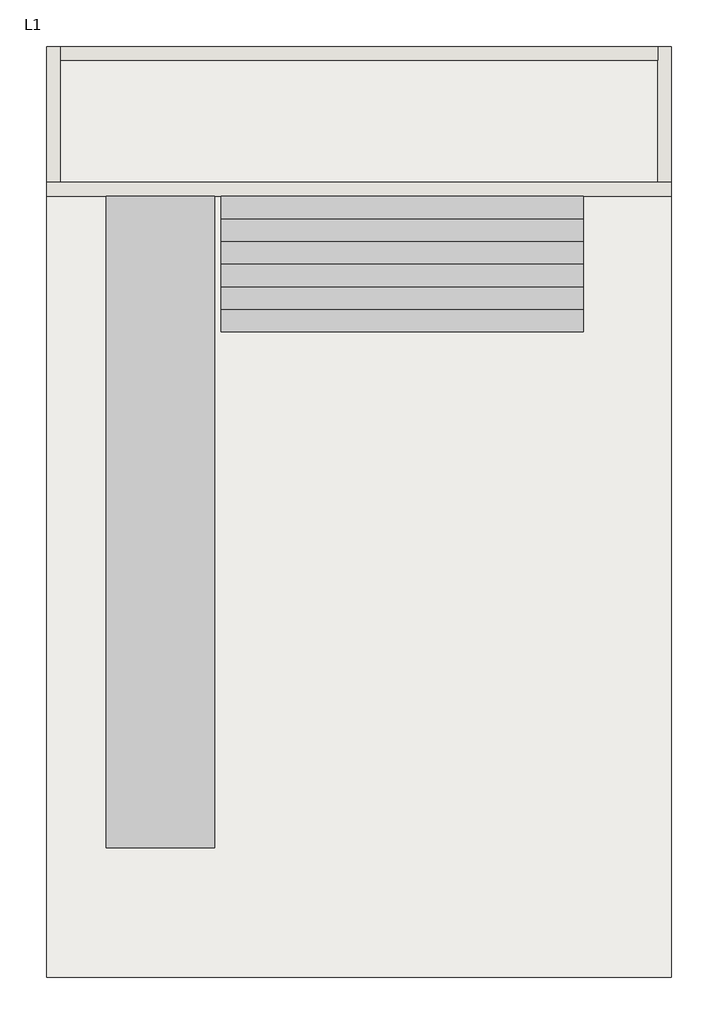
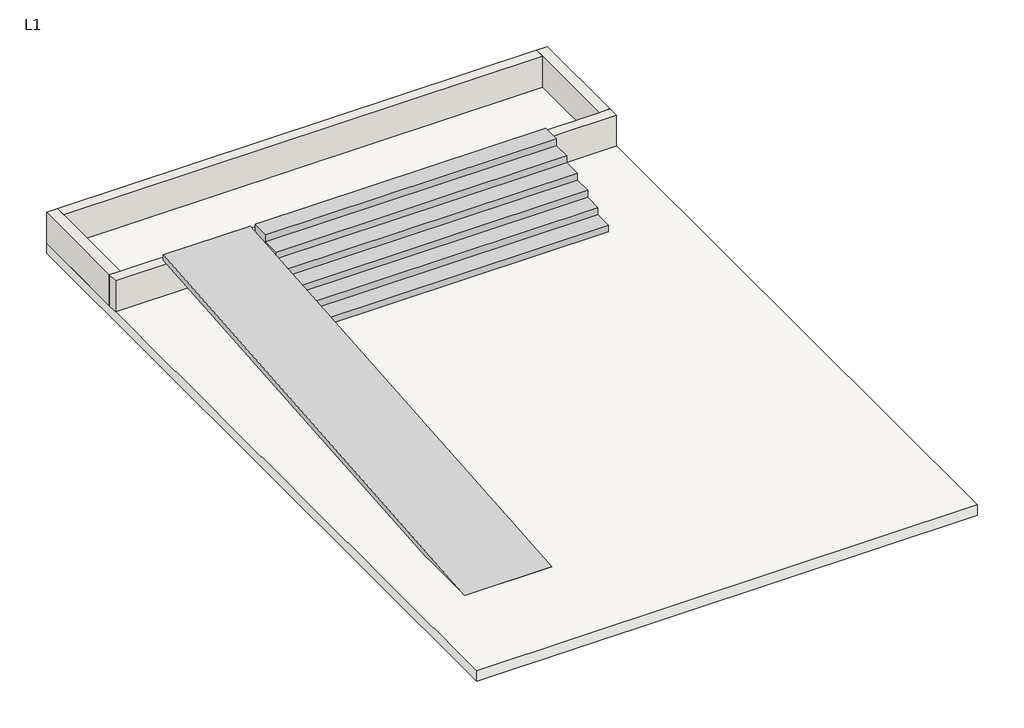
# One storey: 4 walls, 1 ramp, 1 slab, 1 stair flight.
"""IFC4 building model written with IfcOpenShell, lengths in millimetres."""

import ifcopenshell
import ifcopenshell.guid

model = None  # the IFC model being written
_history = None  # IfcOwnerHistory: only IFC2X3 demands one
_inside = {}  # id of a spatial element -> (the spatial element, [elements in it])
_under = {}  # id of a project, library or spatial element -> (it, [spatial elements below it])
_declared = {}  # id of a project -> (the project, [libraries it declares])
_typed = {}  # id of a type object -> (the type object, [elements of that type])
_made_of = {}  # id of a material, layer set ... -> (it, [elements and type objects made of it])


def new_model(schema):
    """Start an empty IFC model of exactly this schema.

    Asked for "IFC4X3", IfcOpenShell would pick the latest addendum, in which some entities
    have other attributes; the version numbers below select the first issue.
    IFC2X3 requires an IfcOwnerHistory on every rooted entity: one is made here for all.
    """
    global model, _history
    if schema == "IFC4X3":
        model = ifcopenshell.file(schema_version=(4, 3, 0, 0))
    else:
        model = ifcopenshell.file(schema=schema)
    _inside.clear()
    _under.clear()
    _declared.clear()
    _typed.clear()
    _made_of.clear()
    _history = None
    if model.schema == "IFC2X3":
        org = make("IfcOrganization", Name="unknown")
        user = make(
            "IfcPersonAndOrganization",
            ThePerson=make("IfcPerson", FamilyName="unknown"),
            TheOrganization=org,
        )
        app = make(
            "IfcApplication",
            ApplicationDeveloper=org,
            Version="unknown",
            ApplicationFullName="unknown",
            ApplicationIdentifier="unknown",
        )
        _history = make(
            "IfcOwnerHistory",
            OwningUser=user,
            OwningApplication=app,
            ChangeAction="ADDED",
            CreationDate=0,
        )
    return model


def make(cls, **values):
    """One entity of the class cls with the attributes given. An attribute that is None is left unset."""
    return model.create_entity(
        cls, **{name: value for name, value in values.items() if value is not None}
    )


def rooted(cls, **values):
    """An entity with a GlobalId (a new one), such as an element, a storey or a relation."""
    return make(cls, GlobalId=ifcopenshell.guid.new(), OwnerHistory=_history, **values)


def si_unit(unit_type, name, prefix=None):
    """IfcSIUnit, for example si_unit("LENGTHUNIT", "METRE", prefix="MILLI")."""
    return make("IfcSIUnit", UnitType=unit_type, Prefix=prefix, Name=name)


def assignment(units):
    """IfcUnitAssignment: the units of a project."""
    return None if units is None else make("IfcUnitAssignment", Units=units)


def point(xyz):
    """IfcCartesianPoint."""
    return None if xyz is None else make("IfcCartesianPoint", Coordinates=xyz)


def direction(xyz):
    """IfcDirection."""
    return None if xyz is None else make("IfcDirection", DirectionRatios=xyz)


def frame(location, z_axis=None, x_axis=None):
    """IfcAxis2Placement3D, a coordinate frame: its origin and axes. An axis left out is left unset."""
    return make(
        "IfcAxis2Placement3D",
        Location=point(location),
        Axis=direction(z_axis),
        RefDirection=direction(x_axis),
    )


def origin():
    """The frame at (0, 0, 0) with its axes left unset."""
    return frame((0.0, 0.0, 0.0))


def origin_with_axes():
    """The frame at (0, 0, 0) with the z axis (0, 0, 1) and the x axis (1, 0, 0) written out."""
    return frame((0.0, 0.0, 0.0), z_axis=(0.0, 0.0, 1.0), x_axis=(1.0, 0.0, 0.0))


def place(relative_to, where):
    """IfcLocalPlacement: puts the frame where relative to a parent placement (None: the world)."""
    return make(
        "IfcLocalPlacement", PlacementRelTo=relative_to, RelativePlacement=where
    )


def context(
    kind, dimensions, precision=None, world=None, true_north=None, identifier=None
):
    """IfcGeometricRepresentationContext, for example the 3D "Model" context."""
    return make(
        "IfcGeometricRepresentationContext",
        ContextIdentifier=identifier,
        ContextType=kind,
        CoordinateSpaceDimension=dimensions,
        Precision=precision,
        WorldCoordinateSystem=world,
        TrueNorth=true_north,
    )


def project(units=None, contexts=None):
    """IfcProject with its units and contexts."""
    return rooted(
        "IfcProject",
        Name="project",
        RepresentationContexts=contexts,
        UnitsInContext=assignment(units),
    )


def spatial(cls, under=None, at=None, **own):
    """A site, building, storey or space (cls), placed at a placement, below another one or the project."""
    s = rooted(cls, ObjectPlacement=at, **own)
    if under is not None:
        _under.setdefault(under.id(), (under, []))[1].append(s)
    return s


def polyline(points):
    """IfcPolyline through the points."""
    return make("IfcPolyline", Points=[point(p) for p in points])


def outline(outer, holes=None, kind="AREA"):
    """IfcArbitraryClosedProfileDef: a profile drawn as a closed curve; with holes, ...WithVoids."""
    if holes is None:
        return make("IfcArbitraryClosedProfileDef", ProfileType=kind, OuterCurve=outer)
    return make(
        "IfcArbitraryProfileDefWithVoids",
        ProfileType=kind,
        OuterCurve=outer,
        InnerCurves=holes,
    )


def extrude(swept, where, along, depth):
    """IfcExtrudedAreaSolid: the profile swept, set in the frame where, extruded along a direction by depth."""
    return make(
        "IfcExtrudedAreaSolid",
        SweptArea=swept,
        Position=where,
        ExtrudedDirection=direction(along),
        Depth=depth,
    )


def faces_of(points, faces, orient=None, outer=None):
    """IfcFace entities. A face is a list of loops; a loop is a list of indices into points, from 0.

    orient and outer hold one flag for each loop. By default every Orientation is true, the
    first loop of a face is its IfcFaceOuterBound and the others are IfcFaceBound.
    """
    made = []
    for i, loops in enumerate(faces):
        bounds = []
        for j, loop in enumerate(loops):
            is_outer = j == 0 if outer is None else outer[i][j]
            bounds.append(
                make(
                    "IfcFaceOuterBound" if is_outer else "IfcFaceBound",
                    Bound=make("IfcPolyLoop", Polygon=[points[k] for k in loop]),
                    Orientation=True if orient is None else orient[i][j],
                )
            )
        made.append(make("IfcFace", Bounds=bounds))
    return made


def faceted_brep(points, faces, orient=None, outer=None, voids=None):
    """IfcFacetedBrep: a solid bounded by flat faces; with voids (closed shells), ...WithVoids."""
    shared = [point(p) for p in points]
    hull = make("IfcClosedShell", CfsFaces=faces_of(shared, faces, orient, outer))
    if voids is None:
        return make("IfcFacetedBrep", Outer=hull)
    return make(
        "IfcFacetedBrepWithVoids",
        Outer=hull,
        Voids=[
            make(cls, CfsFaces=faces_of(shared, fs, o, b)) for cls, fs, o, b in voids
        ],
    )


def shape(context_of_items, identifier, shape_type, items):
    """IfcShapeRepresentation: the items that make up one representation, for example the "Body"."""
    return make(
        "IfcShapeRepresentation",
        ContextOfItems=context_of_items,
        RepresentationIdentifier=identifier,
        RepresentationType=shape_type,
        Items=items,
    )


def source(mapping_origin, context_of_items, identifier, shape_type, items):
    """IfcRepresentationMap: a shape defined once, which mapped items show again and again."""
    return make(
        "IfcRepresentationMap",
        MappingOrigin=mapping_origin,
        MappedRepresentation=shape(context_of_items, identifier, shape_type, items),
    )


def transform(
    local_origin,
    x_axis=None,
    y_axis=None,
    z_axis=None,
    scale=None,
    scale2=None,
    scale3=None,
    uniform=True,
):
    """IfcCartesianTransformationOperator3D, or its non-uniform kind. x_axis, y_axis, z_axis: its Axis1, 2, 3."""
    if uniform:
        return make(
            "IfcCartesianTransformationOperator3D",
            Axis1=direction(x_axis),
            Axis2=direction(y_axis),
            LocalOrigin=point(local_origin),
            Scale=scale,
            Axis3=direction(z_axis),
        )
    return make(
        "IfcCartesianTransformationOperator3DnonUniform",
        Axis1=direction(x_axis),
        Axis2=direction(y_axis),
        LocalOrigin=point(local_origin),
        Scale=scale,
        Axis3=direction(z_axis),
        Scale2=scale2,
        Scale3=scale3,
    )


def mapped(mapping_source, mapping_target):
    """IfcMappedItem: shows the shape of a source again, moved by a transform."""
    return make(
        "IfcMappedItem", MappingSource=mapping_source, MappingTarget=mapping_target
    )


def made_of(thing, what):
    """Note that an element or type object is made of a material, layer set ...; save() writes the relation."""
    if what is not None:
        _made_of.setdefault(what.id(), (what, []))[1].append(thing)
    return thing


def element(
    cls,
    number,
    at=None,
    inside=None,
    cuts=None,
    type_object=None,
    material=None,
    context=None,
    identifier="Body",
    shape_type=None,
    held_by="IfcProductDefinitionShape",
    body=None,
    shapes=None,
    **own,
):
    """One element of the class cls, such as IfcWall. Its Tag is "e" and its number.

    at: its placement. inside: the storey or other place that contains it. cuts: it is an
    opening in that element (IfcRelVoidsElement). A single representation is given by context,
    identifier, shape_type and body (its items); several are given by shapes. held_by: the class
    of the entity that holds the representations. save() writes the other relations.
    """
    e = rooted(cls, Tag="e%d" % number, ObjectPlacement=at, **own)
    if body is not None:
        shapes = [shape(context, identifier, shape_type, body)]
    if shapes is not None:
        e.Representation = make(held_by, Representations=shapes)
    if inside is not None:
        _inside.setdefault(inside.id(), (inside, []))[1].append(e)
    if cuts is not None:
        rooted(
            "IfcRelVoidsElement", RelatingBuildingElement=cuts, RelatedOpeningElement=e
        )
    if type_object is not None:
        _typed.setdefault(type_object.id(), (type_object, []))[1].append(e)
    return made_of(e, material)


def aggregate(whole, parts):
    """IfcRelAggregates: a whole, such as a stair, and the parts it consists of."""
    return rooted("IfcRelAggregates", RelatingObject=whole, RelatedObjects=parts)


def save(model, path):
    """Write the relations noted so far, then the file.

    IfcRelAggregates (storeys below a building ...), IfcRelContainedInSpatialStructure (elements
    in a storey), IfcRelDefinesByType, IfcRelAssociatesMaterial and IfcRelDeclares: one each for
    every whole, place, type object, material and project.
    """
    for whole, parts in _under.values():
        aggregate(whole, parts)
    for where, things in _inside.values():
        rooted(
            "IfcRelContainedInSpatialStructure",
            RelatedElements=things,
            RelatingStructure=where,
        )
    for kind, things in _typed.values():
        rooted("IfcRelDefinesByType", RelatedObjects=things, RelatingType=kind)
    for what, things in _made_of.values():
        rooted("IfcRelAssociatesMaterial", RelatedObjects=things, RelatingMaterial=what)
    for by, libraries in _declared.values():
        rooted("IfcRelDeclares", RelatingContext=by, RelatedDefinitions=libraries)
    model.write(path)


def ramp_1_51a07ffc(model_context):
    return source(origin(), model_context, "Body", "SweptSolid", [
        extrude(outline(polyline([(-8058.4292912, 0.0), (-858.4292912, 600.0), (-858.4292912, 524.7400339), (-8058.4292912, -75.2599661), (-8058.4292912, 0.0)])), frame((-599.8488078, 0.0, 0.0), z_axis=(1.0, 0.0, 0.0), x_axis=(0.0, 1.0, 0.0)), (0.0, 0.0, 1.0), 1200.0),
    ])


model = new_model("IFC4")

# Units and contexts
model_context = context("Model", 3, world=origin())
ifc_project = project(units=[si_unit("LENGTHUNIT", "METRE", prefix="MILLI")], contexts=[model_context])

# Site, building, storey
site = spatial("IfcSite", under=ifc_project)
building = spatial("IfcBuilding", under=site)
storey = spatial("IfcBuildingStorey", under=building, Name="L1", Elevation=0.0)

# Ramp
placement = place(None, origin())
ramp_1_shape = ramp_1_51a07ffc(model_context)
element("IfcRamp", 1, ObjectType="Ramp 1", at=placement, inside=storey, context=model_context, shape_type="MappedRepresentation", body=[
    mapped(ramp_1_shape, transform((0.0, 0.0, 0.0), x_axis=(1.0, 0.0, 0.0), y_axis=(0.0, 1.0, 0.0), z_axis=(0.0, 0.0, 1.0))),
])

# Slab
element("IfcSlab", 2, ObjectType="Concrete 150mm", at=placement, inside=storey, context=model_context, shape_type="SweptSolid", body=[
    extrude(outline(polyline([(5643.2318, -9483.4292912), (-1256.7682, -9483.4292912), (-1256.7682, 791.5707088), (5643.2318, 791.5707088), (5643.2318, -9483.4292912)])), frame((0.0, 0.0, -150.0), z_axis=(0.0, 0.0, 1.0), x_axis=(1.0, 0.0, 0.0)), (0.0, 0.0, 1.0), 150.0),
])

# Stair flight
element("IfcStairFlight", 3, ObjectType="M_Monolithic Run", at=placement, inside=storey, context=model_context, shape_type="Brep", body=[
    faceted_brep([(670.1511922, -2108.4292912, 100.0), (670.1511922, -2358.4292912, 100.0), (4670.1511922, -2358.4292912, 100.0), (4670.1511922, -2108.4292912, 100.0), (670.1511922, -2108.4292912, 0.0), (670.1511922, -2358.4292912, 0.0), (4670.1511922, -2358.4292912, 0.0), (4670.1511922, -2108.4292912, 0.0), (670.1511922, -1858.4292912, 200.0), (670.1511922, -2108.4292912, 200.0), (4670.1511922, -2108.4292912, 200.0), (4670.1511922, -1858.4292912, 200.0), (670.1511922, -1858.4292912, 38.4450558), (670.1511922, -1954.5419306, 0.0), (4670.1511922, -1954.5419306, 0.0), (4670.1511922, -1858.4292912, 38.4450558), (670.1511922, -1608.4292912, 300.0), (670.1511922, -1858.4292912, 300.0), (4670.1511922, -1858.4292912, 300.0), (4670.1511922, -1608.4292912, 300.0), (670.1511922, -1608.4292912, 138.4450558), (4670.1511922, -1608.4292912, 138.4450558), (670.1511922, -1358.4292912, 400.0), (670.1511922, -1608.4292912, 400.0), (4670.1511922, -1608.4292912, 400.0), (4670.1511922, -1358.4292912, 400.0), (670.1511922, -1358.4292912, 238.4450558), (4670.1511922, -1358.4292912, 238.4450558), (670.1511922, -1108.4292912, 500.0), (670.1511922, -1358.4292912, 500.0), (4670.1511922, -1358.4292912, 500.0), (4670.1511922, -1108.4292912, 500.0), (670.1511922, -1108.4292912, 338.4450558), (4670.1511922, -1108.4292912, 338.4450558), (670.1511922, -858.4292912, 600.0), (670.1511922, -1108.4292912, 600.0), (4670.1511922, -1108.4292912, 600.0), (4670.1511922, -858.4292912, 600.0), (670.1511922, -858.4292912, 438.4450558), (4670.1511922, -858.4292912, 438.4450558)], [[[0, 1, 2, 3]], [[1, 0, 4, 5]], [[2, 1, 5, 6]], [[3, 2, 6, 7]], [[8, 9, 10, 11]], [[4, 0, 9, 8, 12, 13]], [[0, 3, 10, 9]], [[3, 7, 14, 15, 11, 10]], [[16, 17, 18, 19]], [[17, 16, 20, 12, 8]], [[8, 11, 18, 17]], [[19, 18, 11, 15, 21]], [[22, 23, 24, 25]], [[23, 22, 26, 20, 16]], [[16, 19, 24, 23]], [[25, 24, 19, 21, 27]], [[28, 29, 30, 31]], [[29, 28, 32, 26, 22]], [[22, 25, 30, 29]], [[31, 30, 25, 27, 33]], [[34, 35, 36, 37]], [[35, 34, 38, 32, 28]], [[28, 31, 36, 35]], [[37, 36, 31, 33, 39]], [[34, 37, 39, 38]], [[5, 4, 13, 14, 7, 6]], [[14, 13, 12, 20, 26, 32, 38, 39, 33, 27, 21, 15]]]),
])

# Walls
element("IfcWall", 4, ObjectType="Generic - 150mm", at=placement, inside=storey, context=model_context, shape_type="Brep", body=[
    faceted_brep([(-1256.7682, -858.4292912, 0.0), (5643.2318, -858.4292912, 0.0), (5643.2318, -858.4292912, 450.0), (-1256.7682, -858.4292912, 450.0), (-1256.7682, -708.4292912, 0.0), (-1256.7682, -708.4292912, 450.0), (-1106.7682, -708.4292912, 450.0), (5493.2318, -708.4292912, 450.0), (5643.2318, -708.4292912, 450.0), (5643.2318, -708.4292912, 0.0), (5493.2318, -708.4292912, 0.0), (-1106.7682, -708.4292912, 0.0)], [[[0, 1, 2, 3]], [[4, 5, 6, 7, 8, 9, 10, 11]], [[1, 0, 4, 11, 10, 9]], [[3, 2, 8, 7, 6, 5]], [[0, 3, 5, 4]], [[2, 1, 9, 8]]]),
])
element("IfcWall", 5, ObjectType="Generic - 150mm", at=placement, inside=storey, context=model_context, shape_type="Brep", body=[
    faceted_brep([(-1106.7682, -708.4292912, 0.0), (-1106.7682, 641.5707088, 0.0), (-1106.7682, 791.5707088, 0.0), (-1106.7682, 791.5707088, 450.0), (-1106.7682, 641.5707088, 450.0), (-1106.7682, -708.4292912, 450.0), (-1256.7682, -708.4292912, 0.0), (-1256.7682, -708.4292912, 450.0), (-1256.7682, 791.5707088, 450.0), (-1256.7682, 791.5707088, 0.0)], [[[0, 1, 2, 3, 4, 5]], [[6, 7, 8, 9]], [[2, 1, 0, 6, 9]], [[5, 4, 3, 8, 7]], [[0, 5, 7, 6]], [[3, 2, 9, 8]]]),
])
element("IfcWall", 6, ObjectType="Generic - 150mm", at=placement, inside=storey, context=model_context, shape_type="Brep", body=[
    faceted_brep([(5643.2318, -708.4292912, 0.0), (5643.2318, 791.5707088, 0.0), (5643.2318, 791.5707088, 450.0), (5643.2318, -708.4292912, 450.0), (5493.2318, -708.4292912, 0.0), (5493.2318, -708.4292912, 450.0), (5493.2318, 641.5707088, 450.0), (5493.2318, 791.5707088, 450.0), (5493.2318, 791.5707088, 0.0), (5493.2318, 641.5707088, 0.0)], [[[0, 1, 2, 3]], [[4, 5, 6, 7, 8, 9]], [[1, 0, 4, 9, 8]], [[3, 2, 7, 6, 5]], [[0, 3, 5, 4]], [[2, 1, 8, 7]]]),
])
element("IfcWall", 7, ObjectType="Generic - 150mm", at=placement, inside=storey, context=model_context, shape_type="SweptSolid", body=[
    extrude(outline(polyline([(5493.2318, 641.5707088), (-1106.7682, 641.5707088), (-1106.7682, 791.5707088), (5493.2318, 791.5707088), (5493.2318, 641.5707088)])), origin_with_axes(), (0.0, 0.0, 1.0), 450.0),
])

save(model, "model.ifc")

# Revit data of these elements
# Project information
#   Organization Name = "Organization Name"
#   Organization Description = "Organization Description"
#   Building Name = "Building Name"
#   Project Issue Date = "Issue Date"
#   Project Status = "Project Status"
#   Client Name = "Client Name"
#   Project Address = "Enter address here\nAddress Line 2"
#   Project Name = "Project Name"
#   Project Number = "Project Number"
# Type "Ramp 1"
#   built-in parameter 1008304 = 0.246063 (stored number, unit not read)
#   built-in parameter 1008303 = 30 (stored number, unit not read)
#   built-in parameter 1008301 = 12 (stored number, unit not read)
#   Function = 0
# Type "Concrete 150mm"
#   Description = "Concrete Floor, 100mm thick, Interior Function"
#   Type Mark = "SF01"
#   Function = 0
#   Layers, outside or top first: 150 mm "Concrete, Cast-in-Place gray" (function 1)
# Type "Generic - 150mm"
#   Description = "Generic Wall (Material By Category), 150mm thick"
#   Type Mark = "G04"
#   Layers, outside or top first: 150 mm no material (function 1)
# Element 1 (IfcRamp, "Ramp 1")
#   built-in parameter 1007275 = "DN"
#   built-in parameter 1007272 = "UP"
#   Width = 1200 mm
#   built-in parameter 1007276 = 1
#   built-in parameter 1007274 = 1
#   built-in parameter 1007273 = 1
#   built-in parameter 1007271 = 1
#   Phase Created = New Construction
# Element 2 (IfcSlab, "Concrete 150mm")
#   Height Offset From Level = 0 mm
#   Phase Created = New Construction
#   Materials on its faces: "Concrete, Cast-in-Place gray"
# Element 3 (IfcStairFlight, "M_Monolithic Run")
#   Phase Created = New Construction
# Element 4 (IfcWall, "Generic - 150mm")
#   Top Offset = 0 mm
#   Base Offset = 0 mm
#   wall height = 600 mm
#   Phase Created = New Construction
#   Base Constraint = L1
#   Top Constraint = L2
#   Materials on its faces: "Default Wall"
# Elements 5, 6, 7 (IfcWall, "Generic - 150mm")
#   Top Offset = 0 mm
#   Base Offset = 0 mm
#   Unconnected Height = 450 mm
#   wall height = 450 mm
#   Phase Created = New Construction
#   Base Constraint = L1
#   Materials on its faces: "Default Wall"
# Materials
#   "Concrete, Cast-in-Place gray": class "Concrete", colour RGB 192 192 192, transparency 0, Description = "Cast-in-place concrete", Cost = 0
#   "Default Wall": class "Miscellaneous", colour RGB 192 192 192, transparency 0, Cost = 0
